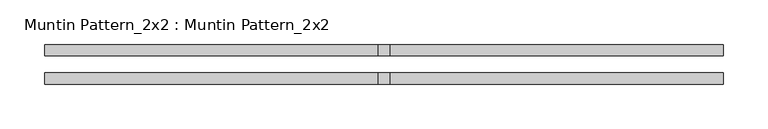
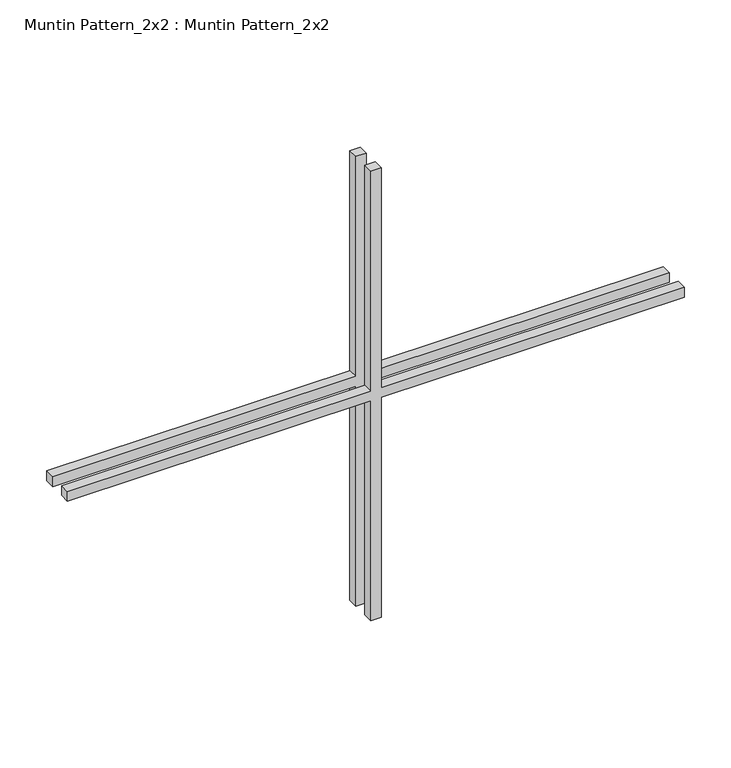
"""IFC4 building model written with IfcOpenShell, lengths in millimetres: proxy geometry, Muntin Pattern_2x2 : Muntin Pattern_2x2."""

import ifcopenshell
import ifcopenshell.guid

model = None  # the IFC model being written
_history = None  # IfcOwnerHistory: only IFC2X3 demands one
_inside = {}  # id of a spatial element -> (the spatial element, [elements in it])
_under = {}  # id of a project, library or spatial element -> (it, [spatial elements below it])
_declared = {}  # id of a project -> (the project, [libraries it declares])
_typed = {}  # id of a type object -> (the type object, [elements of that type])
_made_of = {}  # id of a material, layer set ... -> (it, [elements and type objects made of it])


def new_model(schema):
    """Start an empty IFC model of exactly this schema.

    Asked for "IFC4X3", IfcOpenShell would pick the latest addendum, in which some entities
    have other attributes; the version numbers below select the first issue.
    IFC2X3 requires an IfcOwnerHistory on every rooted entity: one is made here for all.
    """
    global model, _history
    if schema == "IFC4X3":
        model = ifcopenshell.file(schema_version=(4, 3, 0, 0))
    else:
        model = ifcopenshell.file(schema=schema)
    _inside.clear()
    _under.clear()
    _declared.clear()
    _typed.clear()
    _made_of.clear()
    _history = None
    if model.schema == "IFC2X3":
        org = make("IfcOrganization", Name="unknown")
        user = make(
            "IfcPersonAndOrganization",
            ThePerson=make("IfcPerson", FamilyName="unknown"),
            TheOrganization=org,
        )
        app = make(
            "IfcApplication",
            ApplicationDeveloper=org,
            Version="unknown",
            ApplicationFullName="unknown",
            ApplicationIdentifier="unknown",
        )
        _history = make(
            "IfcOwnerHistory",
            OwningUser=user,
            OwningApplication=app,
            ChangeAction="ADDED",
            CreationDate=0,
        )
    return model


def make(cls, **values):
    """One entity of the class cls with the attributes given. An attribute that is None is left unset."""
    return model.create_entity(
        cls, **{name: value for name, value in values.items() if value is not None}
    )


def rooted(cls, **values):
    """An entity with a GlobalId (a new one), such as an element, a storey or a relation."""
    return make(cls, GlobalId=ifcopenshell.guid.new(), OwnerHistory=_history, **values)


def si_unit(unit_type, name, prefix=None):
    """IfcSIUnit, for example si_unit("LENGTHUNIT", "METRE", prefix="MILLI")."""
    return make("IfcSIUnit", UnitType=unit_type, Prefix=prefix, Name=name)


def assignment(units):
    """IfcUnitAssignment: the units of a project."""
    return None if units is None else make("IfcUnitAssignment", Units=units)


def point(xyz):
    """IfcCartesianPoint."""
    return None if xyz is None else make("IfcCartesianPoint", Coordinates=xyz)


def direction(xyz):
    """IfcDirection."""
    return None if xyz is None else make("IfcDirection", DirectionRatios=xyz)


def frame(location, z_axis=None, x_axis=None):
    """IfcAxis2Placement3D, a coordinate frame: its origin and axes. An axis left out is left unset."""
    return make(
        "IfcAxis2Placement3D",
        Location=point(location),
        Axis=direction(z_axis),
        RefDirection=direction(x_axis),
    )


def origin():
    """The frame at (0, 0, 0) with its axes left unset."""
    return frame((0.0, 0.0, 0.0))


def place(relative_to, where):
    """IfcLocalPlacement: puts the frame where relative to a parent placement (None: the world)."""
    return make(
        "IfcLocalPlacement", PlacementRelTo=relative_to, RelativePlacement=where
    )


def context(
    kind, dimensions, precision=None, world=None, true_north=None, identifier=None
):
    """IfcGeometricRepresentationContext, for example the 3D "Model" context."""
    return make(
        "IfcGeometricRepresentationContext",
        ContextIdentifier=identifier,
        ContextType=kind,
        CoordinateSpaceDimension=dimensions,
        Precision=precision,
        WorldCoordinateSystem=world,
        TrueNorth=true_north,
    )


def project(units=None, contexts=None):
    """IfcProject with its units and contexts."""
    return rooted(
        "IfcProject",
        Name="project",
        RepresentationContexts=contexts,
        UnitsInContext=assignment(units),
    )


def spatial(cls, under=None, at=None, **own):
    """A site, building, storey or space (cls), placed at a placement, below another one or the project."""
    s = rooted(cls, ObjectPlacement=at, **own)
    if under is not None:
        _under.setdefault(under.id(), (under, []))[1].append(s)
    return s


def polyline(points):
    """IfcPolyline through the points."""
    return make("IfcPolyline", Points=[point(p) for p in points])


def outline(outer, holes=None, kind="AREA"):
    """IfcArbitraryClosedProfileDef: a profile drawn as a closed curve; with holes, ...WithVoids."""
    if holes is None:
        return make("IfcArbitraryClosedProfileDef", ProfileType=kind, OuterCurve=outer)
    return make(
        "IfcArbitraryProfileDefWithVoids",
        ProfileType=kind,
        OuterCurve=outer,
        InnerCurves=holes,
    )


def extrude(swept, where, along, depth):
    """IfcExtrudedAreaSolid: the profile swept, set in the frame where, extruded along a direction by depth."""
    return make(
        "IfcExtrudedAreaSolid",
        SweptArea=swept,
        Position=where,
        ExtrudedDirection=direction(along),
        Depth=depth,
    )


def shape(context_of_items, identifier, shape_type, items):
    """IfcShapeRepresentation: the items that make up one representation, for example the "Body"."""
    return make(
        "IfcShapeRepresentation",
        ContextOfItems=context_of_items,
        RepresentationIdentifier=identifier,
        RepresentationType=shape_type,
        Items=items,
    )


def source(mapping_origin, context_of_items, identifier, shape_type, items):
    """IfcRepresentationMap: a shape defined once, which mapped items show again and again."""
    return make(
        "IfcRepresentationMap",
        MappingOrigin=mapping_origin,
        MappedRepresentation=shape(context_of_items, identifier, shape_type, items),
    )


def transform(
    local_origin,
    x_axis=None,
    y_axis=None,
    z_axis=None,
    scale=None,
    scale2=None,
    scale3=None,
    uniform=True,
):
    """IfcCartesianTransformationOperator3D, or its non-uniform kind. x_axis, y_axis, z_axis: its Axis1, 2, 3."""
    if uniform:
        return make(
            "IfcCartesianTransformationOperator3D",
            Axis1=direction(x_axis),
            Axis2=direction(y_axis),
            LocalOrigin=point(local_origin),
            Scale=scale,
            Axis3=direction(z_axis),
        )
    return make(
        "IfcCartesianTransformationOperator3DnonUniform",
        Axis1=direction(x_axis),
        Axis2=direction(y_axis),
        LocalOrigin=point(local_origin),
        Scale=scale,
        Axis3=direction(z_axis),
        Scale2=scale2,
        Scale3=scale3,
    )


def mapped(mapping_source, mapping_target):
    """IfcMappedItem: shows the shape of a source again, moved by a transform."""
    return make(
        "IfcMappedItem", MappingSource=mapping_source, MappingTarget=mapping_target
    )


def made_of(thing, what):
    """Note that an element or type object is made of a material, layer set ...; save() writes the relation."""
    if what is not None:
        _made_of.setdefault(what.id(), (what, []))[1].append(thing)
    return thing


def element(
    cls,
    number,
    at=None,
    inside=None,
    cuts=None,
    type_object=None,
    material=None,
    context=None,
    identifier="Body",
    shape_type=None,
    held_by="IfcProductDefinitionShape",
    body=None,
    shapes=None,
    **own,
):
    """One element of the class cls, such as IfcWall. Its Tag is "e" and its number.

    at: its placement. inside: the storey or other place that contains it. cuts: it is an
    opening in that element (IfcRelVoidsElement). A single representation is given by context,
    identifier, shape_type and body (its items); several are given by shapes. held_by: the class
    of the entity that holds the representations. save() writes the other relations.
    """
    e = rooted(cls, Tag="e%d" % number, ObjectPlacement=at, **own)
    if body is not None:
        shapes = [shape(context, identifier, shape_type, body)]
    if shapes is not None:
        e.Representation = make(held_by, Representations=shapes)
    if inside is not None:
        _inside.setdefault(inside.id(), (inside, []))[1].append(e)
    if cuts is not None:
        rooted(
            "IfcRelVoidsElement", RelatingBuildingElement=cuts, RelatedOpeningElement=e
        )
    if type_object is not None:
        _typed.setdefault(type_object.id(), (type_object, []))[1].append(e)
    return made_of(e, material)


def aggregate(whole, parts):
    """IfcRelAggregates: a whole, such as a stair, and the parts it consists of."""
    return rooted("IfcRelAggregates", RelatingObject=whole, RelatedObjects=parts)


def save(model, path):
    """Write the relations noted so far, then the file.

    IfcRelAggregates (storeys below a building ...), IfcRelContainedInSpatialStructure (elements
    in a storey), IfcRelDefinesByType, IfcRelAssociatesMaterial and IfcRelDeclares: one each for
    every whole, place, type object, material and project.
    """
    for whole, parts in _under.values():
        aggregate(whole, parts)
    for where, things in _inside.values():
        rooted(
            "IfcRelContainedInSpatialStructure",
            RelatedElements=things,
            RelatingStructure=where,
        )
    for kind, things in _typed.values():
        rooted("IfcRelDefinesByType", RelatedObjects=things, RelatingType=kind)
    for what, things in _made_of.values():
        rooted("IfcRelAssociatesMaterial", RelatedObjects=things, RelatingMaterial=what)
    for by, libraries in _declared.values():
        rooted("IfcRelDeclares", RelatingContext=by, RelatedDefinitions=libraries)
    model.write(path)


def muntin_pattern_2x2_muntin_pattern_2x2_c1e6ccc8(model_context):
    return source(origin(), model_context, "Body", "SweptSolid", [
        extrude(outline(polyline([(300.0375, -6.35), (300.0375, -381.0), (287.3375, -381.0), (287.3375, -6.35), (0.0, -6.35), (0.0, 6.35), (287.3375, 6.35), (287.3375, 381.0), (300.0375, 381.0), (300.0375, 6.35), (587.375, 6.35), (587.375, -6.35), (300.0375, -6.35)])), frame((0.0, 9.525, 0.0), z_axis=(0.0, 1.0, 0.0), x_axis=(0.0, 0.0, 1.0)), (0.0, 0.0, 1.0), 12.7),
        extrude(outline(polyline([(300.0375, -6.35), (300.0375, -381.0), (287.3375, -381.0), (287.3375, -6.35), (0.0, -6.35), (0.0, 6.35), (287.3375, 6.35), (287.3375, 381.0), (300.0375, 381.0), (300.0375, 6.35), (587.375, 6.35), (587.375, -6.35), (300.0375, -6.35)])), frame((0.0, -22.225, 0.0), z_axis=(0.0, 1.0, 0.0), x_axis=(0.0, 0.0, 1.0)), (0.0, 0.0, 1.0), 12.7),
    ])


if __name__ == "__main__":
    model = new_model("IFC4")
    model_context = context("Model", 3, world=origin())
    ifc_project = project(units=[si_unit("LENGTHUNIT", "METRE", prefix="MILLI")], contexts=[model_context])
    site = spatial("IfcSite", under=ifc_project)
    building = spatial("IfcBuilding", under=site)
    placement = place(None, origin())
    muntin_pattern_2x2_muntin_pattern_2x2_shape = muntin_pattern_2x2_muntin_pattern_2x2_c1e6ccc8(model_context)
    element("IfcBuildingElementProxy", 1, Name="Muntin Pattern_2x2 : Muntin Pattern_2x2", ObjectType="Muntin Pattern_2x2 : Muntin Pattern_2x2", at=placement, inside=building, context=model_context, shape_type="MappedRepresentation", body=[
        mapped(muntin_pattern_2x2_muntin_pattern_2x2_shape, transform((0.0, 0.0, 0.0), x_axis=(1.0, 0.0, 0.0), y_axis=(0.0, 1.0, 0.0), z_axis=(0.0, 0.0, 1.0))),
    ])
    save(model, "model.ifc")

# Revit data of these elements
# Type "Muntin Pattern_2x2 : Muntin Pattern_2x2"
#   Width [instance default] = 4' - 0"
#   Thickness = 0' - 0 1/2"
#   Height [instance default] = 4' - 0"
#   Distance = 0' - 0 3/4"
#   Interior Material [instance default] = none
#   Exterior Material [instance default] = none
#   Default Elevation = 0
# Element 1 (IfcBuildingElementProxy, "Muntin Pattern_2x2 : Muntin Pattern_2x2")
#   Width = 2' - 6"
#   Height = 1' - 11 1/8"
#   Interior Material = Wood - Stained
#   Exterior Material = Clad - White
#   Materials on its faces: "Clad - White", "Wood - Stained"
# Materials
#   "Clad - White": class "Wood", colour RGB 242 242 238, transparency 0, Cost = 0
#   "Wood - Stained": class "Wood", colour RGB 224 178 126, transparency 0, Cost = 0
